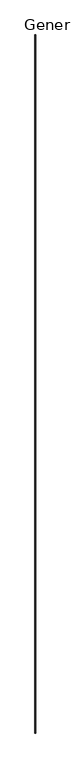
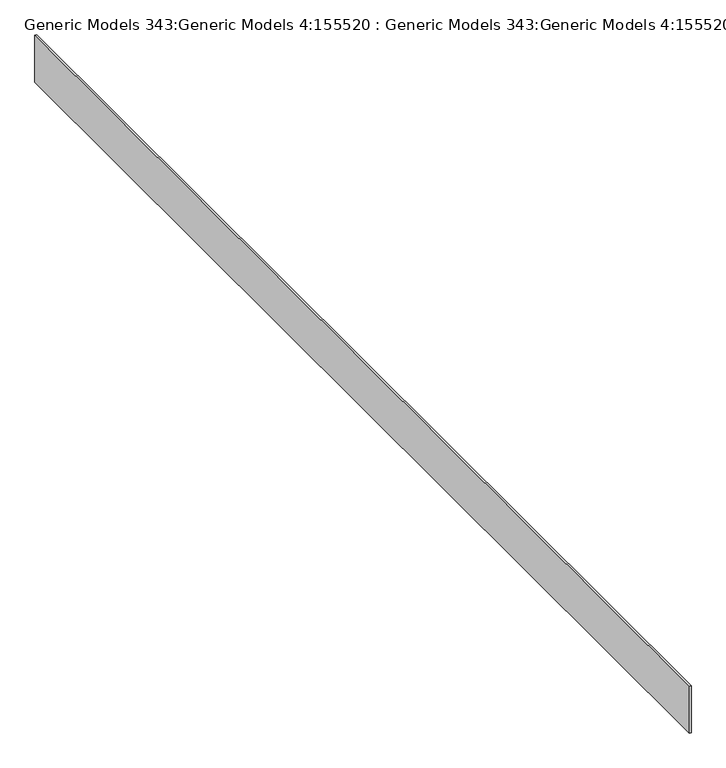
"""IFC4 building model written with IfcOpenShell, lengths in millimetres: proxy geometry, Generic Models 343:Generic Models 4:155520 : Generic Models 343:Generic Models 4:155520."""

from ifc_helpers import new_model, si_unit, frame, origin, place, context, project, spatial, polyline, outline, extrude, source, transform, mapped, element, save


def generic_models_343_generic_models_4_155520_generic_models_e968ca35(model_context):
    return source(origin(), model_context, "Body", "SweptSolid", [
        extrude(outline(polyline([(3927.4671067, -6671.4461219), (3927.4671067, -6689.3043913), (3392.17, -6689.3043913), (3392.17, -6670.9844166), (3908.4171067, -6670.9844166), (3927.4671067, -6671.4461219)])), frame((0.0, -12516.7974793, 0.0), z_axis=(0.0, 1.0, 0.0), x_axis=(0.0, 0.0, 1.0)), (0.0, 0.0, 1.0), 12242.8),
    ])


if __name__ == "__main__":
    model = new_model("IFC4")
    model_context = context("Model", 3, world=origin())
    ifc_project = project(units=[si_unit("LENGTHUNIT", "METRE", prefix="MILLI")], contexts=[model_context])
    site = spatial("IfcSite", under=ifc_project)
    building = spatial("IfcBuilding", under=site)
    placement = place(None, origin())
    generic_models_343_generic_models_4_155520_generic_models_shape = generic_models_343_generic_models_4_155520_generic_models_e968ca35(model_context)
    element("IfcBuildingElementProxy", 1, Name="Generic Models 343:Generic Models 4:155520 : Generic Models 343:Generic Models 4:155520", ObjectType="Generic Models 343:Generic Models 4:155520 : Generic Models 343:Generic Models 4:155520", at=placement, inside=building, context=model_context, shape_type="MappedRepresentation", body=[
        mapped(generic_models_343_generic_models_4_155520_generic_models_shape, transform((0.0, 0.0, 0.0), x_axis=(1.0, 0.0, 0.0), y_axis=(0.0, 1.0, 0.0), z_axis=(0.0, 0.0, 1.0))),
    ])
    save(model, "model.ifc")

# Revit data of these elements
# Type "Generic Models 343:Generic Models 4:155520 : Generic Models 343:Generic Models 4:155520"
#   NameOverride = "Generic Models 343:Generic Models 4:155520"
#   ObjectTypeOverride = "Generic Models 343:Generic Models 4"
#   Reference = "Generic Models 4"
#   Category = "Generic Models"
#   Tag = "155520"
# Element 1 (IfcBuildingElementProxy, "Generic Models 343:Generic Models 4:155520 : Generic Models 343:Generic Models 4:155520")
#   Materials on its faces: "_7/8\" SMOOTH TROWEL EXTERIOR STUCCO (COLOR PER OWNER) 770"
# Materials
#   "_7/8\" SMOOTH TROWEL EXTERIOR STUCCO (COLOR PER OWNER) 770": class "Unassigned", colour RGB 233 233 233, transparency 0
